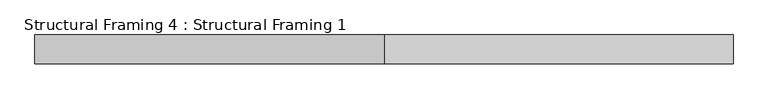
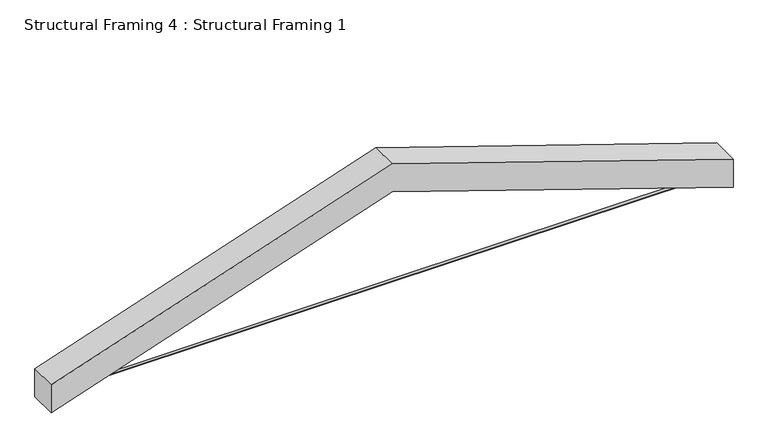
"""IFC4 building model written with IfcOpenShell, lengths in millimetres: beam geometry, Structural Framing 4 : Structural Framing 1."""

from ifc_helpers import new_model, si_unit, point, frame, frame_2d, origin, place, context, project, spatial, polyline, circle_curve, trimmed, segment, composite_curve, outline, extrude, source, transform, mapped, element, save


def structural_framing_4_structural_framing_1_000186f3(model_context):
    return source(origin(), model_context, "Body", "SweptSolid", [
        extrude(outline(composite_curve([segment(trimmed(circle_curve(frame_2d((-1046.4884634, 4984.3019529)), 6.35), [point((-1040.1384634, 4984.3019529))], [point((-1052.8384634, 4984.3019529))], False, "CARTESIAN"), True, "CONTINUOUS"), segment(trimmed(circle_curve(frame_2d((-1046.4884634, 4984.3019529)), 6.35), [point((-1052.8384634, 4984.3019529))], [point((-1040.1384634, 4984.3019529))], False, "CARTESIAN"), True, "CONTINUOUS")], self_intersect=False)), frame((19888.9870052, 0.0, 0.0), z_axis=(1.0, 0.0, 0.0), x_axis=(0.0, 1.0, 0.0)), (0.0, 0.0, 1.0), 3111.5),
        extrude(outline(polyline([(5652.475838, 21444.7370052), (5084.8528105, 19749.2870052), (4937.5315162, 19749.2870052), (5505.1545437, 21444.7370052), (4937.5315162, 23140.1870052), (5084.8528105, 23140.1870052), (5652.475838, 21444.7370052)])), frame((0.0, -1116.3384634, 0.0), z_axis=(0.0, 1.0, 0.0), x_axis=(0.0, 0.0, 1.0)), (0.0, 0.0, 1.0), 139.7),
    ])


if __name__ == "__main__":
    model = new_model("IFC4")
    model_context = context("Model", 3, world=origin())
    ifc_project = project(units=[si_unit("LENGTHUNIT", "METRE", prefix="MILLI")], contexts=[model_context])
    site = spatial("IfcSite", under=ifc_project)
    building = spatial("IfcBuilding", under=site)
    placement = place(None, origin())
    structural_framing_4_structural_framing_1_shape = structural_framing_4_structural_framing_1_000186f3(model_context)
    element("IfcBeam", 1, ObjectType="Structural Framing 4 : Structural Framing 1", at=placement, inside=building, context=model_context, shape_type="MappedRepresentation", body=[
        mapped(structural_framing_4_structural_framing_1_shape, transform((0.0, 0.0, 0.0), x_axis=(1.0, 0.0, 0.0), y_axis=(0.0, 1.0, 0.0), z_axis=(0.0, 0.0, 1.0))),
    ])
    save(model, "model.ifc")

# Revit data of these elements
# Project information
#   Project Issue Date = "03/14/2018"
#   Project Status = "Project Status"
#   Client Name = "Owner"
#   Project Address = "39900 60TH ST BURLINGTON 53105"
#   Project Name = "RIVER VALLEY RANCH"
#   Project Number = "Project Number"
# Element 1 (IfcBeam, "Structural Framing 4 : Structural Framing 1")
#   Materials on its faces: "GLULAM TRUSS W/ CUSTOM GUSSET PLATES", "COLLAR TIE: 1/2\" GALV. ROD"
# Materials
#   "GLULAM TRUSS W/ CUSTOM GUSSET PLATES": class "Generic", colour RGB 206 153 90, transparency 0, Cost = 0
#   "COLLAR TIE: 1/2\" GALV. ROD": class "Generic", colour RGB 49 49 49, transparency 0, Cost = 0
